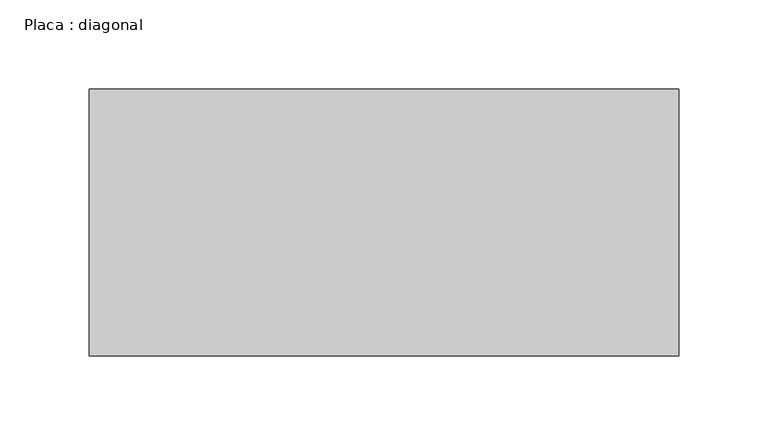
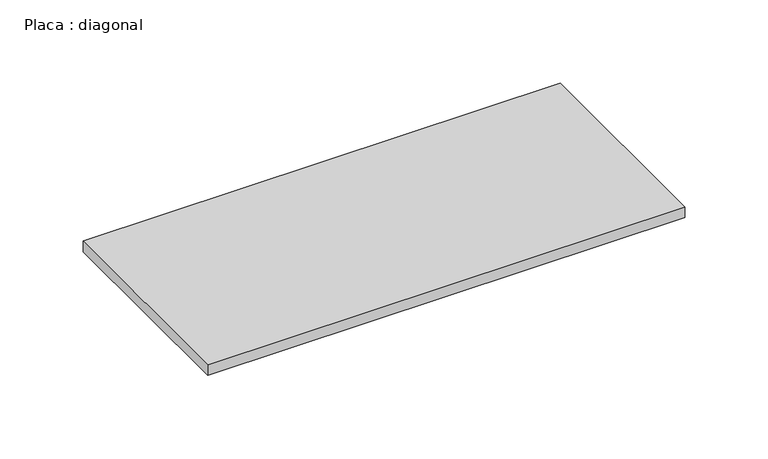
"""IFC4 building model written with IfcOpenShell, lengths in millimetres: beam geometry, Placa : diagonal."""

from ifc_helpers import new_model, si_unit, frame, origin, place, context, project, spatial, polyline, outline, extrude, source, transform, mapped, element, save


def placa_diagonal_5f8fd6b3(model_context):
    return source(origin(), model_context, "Body", "SweptSolid", [
        extrude(outline(polyline([(165.7219053, 75.0), (165.7219053, -75.0), (-165.392588, -75.0), (-165.392588, 75.0), (165.7219053, 75.0)])), frame((0.0, 0.0, -4.0), z_axis=(0.0, 0.0, 1.0), x_axis=(1.0, 0.0, 0.0)), (0.0, 0.0, 1.0), 8.0),
    ])


if __name__ == "__main__":
    model = new_model("IFC4")
    model_context = context("Model", 3, world=origin())
    ifc_project = project(units=[si_unit("LENGTHUNIT", "METRE", prefix="MILLI")], contexts=[model_context])
    site = spatial("IfcSite", under=ifc_project)
    building = spatial("IfcBuilding", under=site)
    placement = place(None, origin())
    placa_diagonal_shape = placa_diagonal_5f8fd6b3(model_context)
    element("IfcBeam", 1, ObjectType="Placa : diagonal", at=placement, inside=building, context=model_context, shape_type="MappedRepresentation", body=[
        mapped(placa_diagonal_shape, transform((0.0, 0.0, 0.0), x_axis=(1.0, 0.0, 0.0), y_axis=(0.0, 1.0, 0.0), z_axis=(0.0, 0.0, 1.0))),
    ])
    save(model, "model.ifc")

# Revit data of these elements
# Type "Placa : diagonal"
#   W = 0
#   Length [instance default] = 1.50 m
#   b = 0.15 m
#   d = 0.008 m
#   A = 0 m²
#   Structural Material [instance default] = Aço, 45-345
# Element 1 (IfcBeam, "Placa : diagonal")
#   Materials on its faces: "Aço, 45-345"
# Materials
#   "Aço, 45-345": class "Metal", colour RGB 247 247 247, transparency 0, Description = "Aço 345 MPa", Cost = 0
